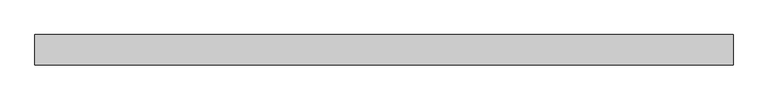
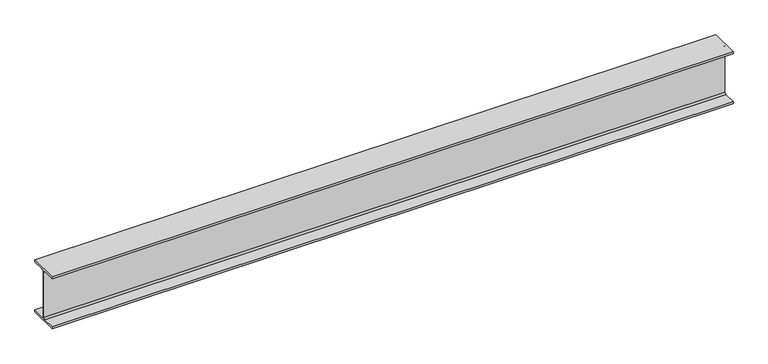
"""IFC4 building model written with IfcOpenShell, lengths in millimetres: beam geometry, Old_Steel Beam_H-KSD3502 : H_SB_ASB_H-200×200x8x12."""

from ifc_helpers import new_model, si_unit, point, frame, frame_2d, origin, place, context, project, spatial, polyline, circle_curve, trimmed, segment, composite_curve, outline, extrude, source, transform, mapped, element, save


def beam_959fe1cf(model_context):
    return source(origin(), model_context, "Body", "SweptSolid", [
        extrude(outline(composite_curve([segment(polyline([(82.5, -141.5), (82.5, -151.7), (-82.5, -151.7), (-82.5, -141.5), (-11.9, -141.5)]), True, "CONTINUOUS"), segment(trimmed(circle_curve(frame_2d((-11.9, -132.6)), 8.9), [point((-11.9, -141.5))], [point((-3.0, -132.6))], True, "CARTESIAN"), True, "CONTINUOUS"), segment(polyline([(-3.0, -132.6), (-3.0, 132.6)]), True, "CONTINUOUS"), segment(trimmed(circle_curve(frame_2d((-11.9, 132.6)), 8.9), [point((-3.0, 132.6))], [point((-11.9, 141.5))], True, "CARTESIAN"), True, "CONTINUOUS"), segment(polyline([(-11.9, 141.5), (-82.5, 141.5), (-82.5, 151.7), (82.5, 151.7), (82.5, 141.5), (11.9, 141.5)]), True, "CONTINUOUS"), segment(trimmed(circle_curve(frame_2d((11.9, 132.6)), 8.9), [point((11.9, 141.5))], [point((3.0, 132.6))], True, "CARTESIAN"), True, "CONTINUOUS"), segment(polyline([(3.0, 132.6), (3.0, -132.6)]), True, "CONTINUOUS"), segment(trimmed(circle_curve(frame_2d((11.9, -132.6)), 8.9), [point((3.0, -132.6))], [point((11.9, -141.5))], True, "CARTESIAN"), True, "CONTINUOUS"), segment(polyline([(11.9, -141.5), (82.5, -141.5)]), True, "CONTINUOUS")], self_intersect=False)), frame((-1951.5443955, 0.0, 0.0), z_axis=(1.0, 0.0, 0.0), x_axis=(0.0, 1.0, 0.0)), (0.0, 0.0, 1.0), 3783.3895896),
    ])


if __name__ == "__main__":
    model = new_model("IFC4")
    model_context = context("Model", 3, world=origin())
    ifc_project = project(units=[si_unit("LENGTHUNIT", "METRE", prefix="MILLI")], contexts=[model_context])
    site = spatial("IfcSite", under=ifc_project)
    building = spatial("IfcBuilding", under=site)
    placement = place(None, origin())
    beam_shape = beam_959fe1cf(model_context)
    element("IfcBeam", 1, ObjectType="Old_Steel Beam_H-KSD3502 : H_SB_ASB_H-200×200x8x12", at=placement, inside=building, context=model_context, shape_type="MappedRepresentation", body=[
        mapped(beam_shape, transform((0.0, 0.0, 0.0), x_axis=(1.0, 0.0, 0.0), y_axis=(0.0, 1.0, 0.0), z_axis=(0.0, 0.0, 1.0))),
    ])
    save(model, "model.ifc")

# Revit data of these elements
# Type "Old_Steel Beam_H-KSD3502 : H_SB_ASB_H-200×200x8x12"
#   Width = 20.0 cm
#   Web Thickness = 0.8 cm
#   Web Fillet = 1.3 cm
#   Warping Constant = 141376.0 cm⁶
#   Torsional Moment of Inertia = 26.2485 cm⁴
#   Torsional Modulus = 1.0 cm³
#   Section Area = 63.53 cm²
#   Plastic Modulus weak axis = 244.0 cm³
#   Plastic Modulus strong axis = 525.0 cm³
#   Perimeter = 1.16 m²/m
#   Nominal Weight = 49.90 kgf/m
#   Moment of Inertia weak axis = 1600.00 cm⁴
#   Moment of Inertia strong axis = 4720.00 cm⁴
#   Height = 20.0 cm
#   Flange Thickness = 1.2 cm
#   Elastic Modulus weak axis = 160.0 cm³
#   Elastic Modulus strong axis = 472.0 cm³
#   Centroid Vertical = 10.0 cm
#   Centroid Horizontal = 10.0 cm
#   Length [instance default] = 1.5240 m
#   Structural Material [instance default] = Steel, 45-345
#   Assembly Code = ""
# Element 1 (IfcBeam, "Old_Steel Beam_H-KSD3502 : H_SB_ASB_H-200×200x8x12")
#   Structural Material = none
# Materials
#   "Steel, 45-345": class "Metal", colour RGB 189 187 185, transparency 0, Description = "Steel 345 MPa", Cost = 0
